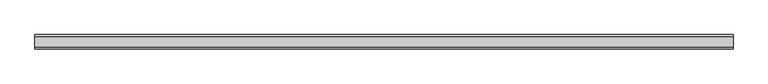
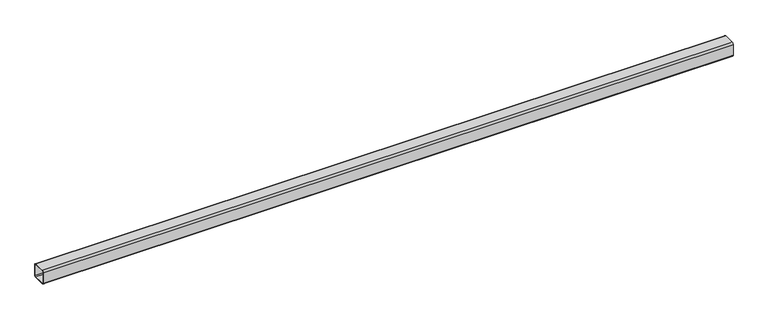
"""IFC4 building model written with IfcOpenShell, lengths in millimetres: beam geometry, Гнутый прямоугольный профиль (Трубы 30245-94) Балки : гнутый прямоуг. проф. 100x6."""

from ifc_helpers import new_model, si_unit, point, frame, frame_2d, origin, place, context, project, spatial, polyline, circle_curve, trimmed, segment, composite_curve, outline, extrude, source, transform, mapped, element, save


def beam_046d7410(model_context):
    return source(origin(), model_context, "Body", "SweptSolid", [
        extrude(outline(composite_curve([segment(polyline([(-38.0, 50.0), (38.0, 50.0)]), True, "CONTINUOUS"), segment(trimmed(circle_curve(frame_2d((38.0, 38.0)), 12.0), [point((38.0, 50.0))], [point((50.0, 38.0))], False, "CARTESIAN"), True, "CONTINUOUS"), segment(polyline([(50.0, 38.0), (50.0, -38.0)]), True, "CONTINUOUS"), segment(trimmed(circle_curve(frame_2d((38.0, -38.0)), 12.0), [point((50.0, -38.0))], [point((38.0, -50.0))], False, "CARTESIAN"), True, "CONTINUOUS"), segment(polyline([(38.0, -50.0), (-38.0, -50.0)]), True, "CONTINUOUS"), segment(trimmed(circle_curve(frame_2d((-38.0, -38.0)), 12.0), [point((-38.0, -50.0))], [point((-50.0, -38.0))], False, "CARTESIAN"), True, "CONTINUOUS"), segment(polyline([(-50.0, -38.0), (-50.0, 38.0)]), True, "CONTINUOUS"), segment(trimmed(circle_curve(frame_2d((-38.0, 38.0)), 12.0), [point((-50.0, 38.0))], [point((-38.0, 50.0))], False, "CARTESIAN"), True, "CONTINUOUS")], self_intersect=False), holes=[composite_curve([segment(trimmed(circle_curve(frame_2d((-38.0, 38.0)), 6.0), [point((-38.0, 44.0))], [point((-44.0, 38.0))], True, "CARTESIAN"), True, "CONTINUOUS"), segment(polyline([(-44.0, 38.0), (-44.0, -38.0)]), True, "CONTINUOUS"), segment(trimmed(circle_curve(frame_2d((-38.0, -38.0)), 6.0), [point((-44.0, -38.0))], [point((-38.0, -44.0))], True, "CARTESIAN"), True, "CONTINUOUS"), segment(polyline([(-38.0, -44.0), (38.0, -44.0)]), True, "CONTINUOUS"), segment(trimmed(circle_curve(frame_2d((38.0, -38.0)), 6.0), [point((38.0, -44.0))], [point((44.0, -38.0))], True, "CARTESIAN"), True, "CONTINUOUS"), segment(polyline([(44.0, -38.0), (44.0, 38.0)]), True, "CONTINUOUS"), segment(trimmed(circle_curve(frame_2d((38.0, 38.0)), 6.0), [point((44.0, 38.0))], [point((38.0, 44.0))], True, "CARTESIAN"), True, "CONTINUOUS"), segment(polyline([(38.0, 44.0), (-38.0, 44.0)]), True, "CONTINUOUS")], self_intersect=False)]), frame((-2400.0, 0.0, 0.0), z_axis=(1.0, 0.0, 0.0), x_axis=(0.0, 1.0, 0.0)), (0.0, 0.0, 1.0), 4800.0),
    ])


if __name__ == "__main__":
    model = new_model("IFC4")
    model_context = context("Model", 3, world=origin())
    ifc_project = project(units=[si_unit("LENGTHUNIT", "METRE", prefix="MILLI")], contexts=[model_context])
    site = spatial("IfcSite", under=ifc_project)
    building = spatial("IfcBuilding", under=site)
    placement = place(None, origin())
    beam_shape = beam_046d7410(model_context)
    element("IfcBeam", 1, ObjectType="Гнутый прямоугольный профиль (Трубы 30245-94) Балки : гнутый прямоуг. проф. 100x6", at=placement, inside=building, context=model_context, shape_type="MappedRepresentation", body=[
        mapped(beam_shape, transform((0.0, 0.0, 0.0), x_axis=(1.0, 0.0, 0.0), y_axis=(0.0, 1.0, 0.0), z_axis=(0.0, 0.0, 1.0))),
    ])
    save(model, "model.ifc")

# Revit data of these elements
# Type "Гнутый прямоугольный профиль (Трубы 30245-94) Балки : гнутый прямоуг. проф. 100x6"
#   ri = 12 mm
#   ra = 6 mm
#   W = 0.173578
#   Vz = 50 mm
#   Vy = 50 mm
#   Vpz = 50 mm
#   Vpy = 50 mm
#   Length [instance default] = 1500 mm
#   bf = 100 mm
#   d = 100 mm
#   tf = 6 mm
#   tw = 6 mm
#   A = 0.00226 m²
#   Structural Material [instance default] = Металл - Сталь - 345 МПa
#   Assembly Code = ""
# Element 1 (IfcBeam, "Гнутый прямоугольный профиль (Трубы 30245-94) Балки : гнутый прямоуг. проф. 100x6")
#   Structural Material = C235
#   Materials on its faces: "C235"
# Materials
#   "Металл - Сталь - 345 МПa": class "Металл", colour RGB 247 247 247, transparency 0
#   "C235": class "Не назначено", colour RGB 0 0 0, transparency 0
